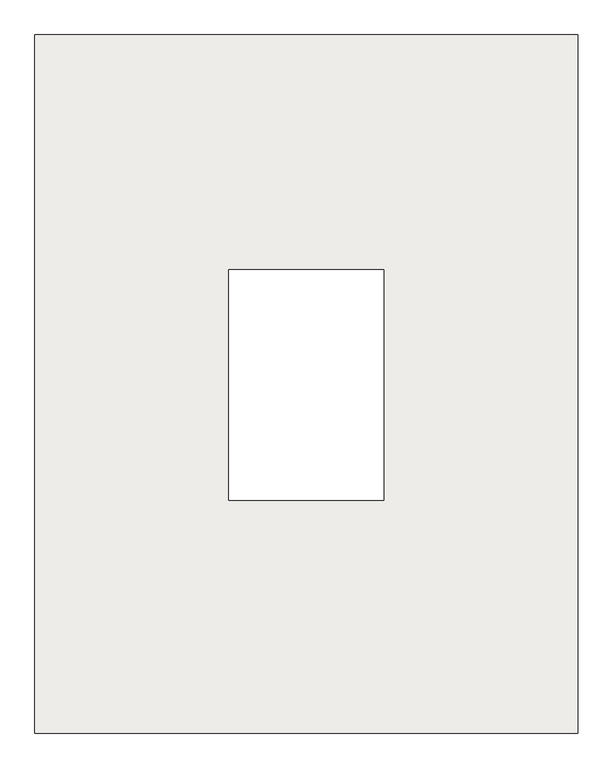
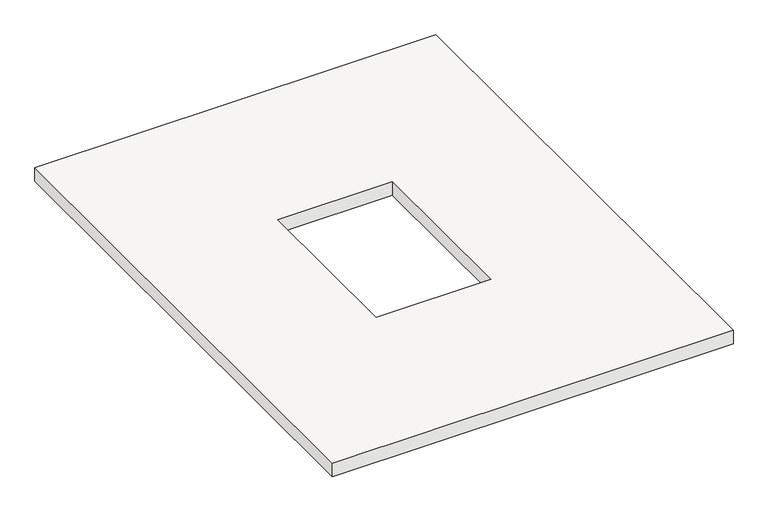
"""IFC4 building model written with IfcOpenShell, lengths in millimetres: slab geometry, Holzdecke."""

from ifc_helpers import new_model, si_unit, origin, origin_with_axes, place, context, project, spatial, polyline, outline, extrude, source, transform, mapped, element, save


def slab_c25f4032(model_context):
    return source(origin(), model_context, "Body", "SweptSolid", [
        extrude(outline(polyline([(0.0, 0.0), (0.0, 18002.8619019), (14000.0, 18002.8619019), (14000.0, 0.0), (0.0, 0.0)]), holes=[polyline([(9000.0, 11952.8619019), (5000.0, 11952.8619019), (5000.0, 6002.8619019), (9000.0, 6002.8619019), (9000.0, 11952.8619019)])]), origin_with_axes(), (0.0, 0.0, 1.0), 500.0),
    ])


if __name__ == "__main__":
    model = new_model("IFC4")
    model_context = context("Model", 3, world=origin())
    ifc_project = project(units=[si_unit("LENGTHUNIT", "METRE", prefix="MILLI")], contexts=[model_context])
    site = spatial("IfcSite", under=ifc_project)
    building = spatial("IfcBuilding", under=site)
    placement = place(None, origin())
    slab_shape = slab_c25f4032(model_context)
    element("IfcSlab", 1, ObjectType="Holzdecke", at=placement, inside=building, context=model_context, shape_type="MappedRepresentation", body=[
        mapped(slab_shape, transform((0.0, 0.0, 0.0), x_axis=(1.0, 0.0, 0.0), y_axis=(0.0, 1.0, 0.0), z_axis=(0.0, 0.0, 1.0))),
    ])
    save(model, "model.ifc")

# Revit data of these elements
# Element 1 (IfcSlab, "Holzdecke")
#   Materials on its faces: "holzschalung"
# Materials
#   "holzschalung": class "Unassigned", colour RGB 128 128 128, transparency 0
